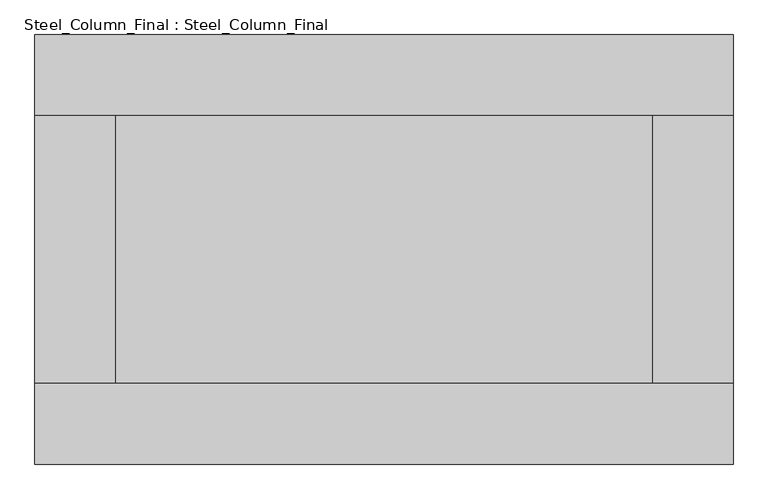
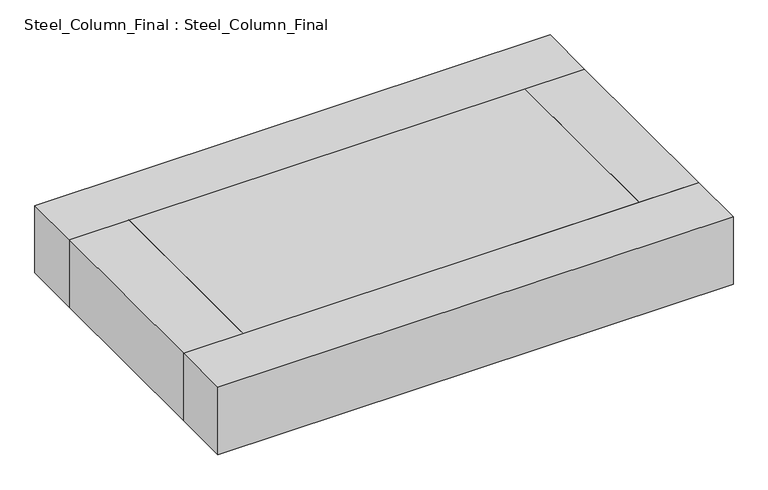
"""IFC4 building model written with IfcOpenShell, lengths in millimetres: proxy geometry, Steel_Column_Final : Steel_Column_Final."""

from ifc_helpers import new_model, si_unit, frame, origin, place, context, project, spatial, polyline, outline, extrude, source, transform, mapped, element, save


def steel_column_final_steel_column_final_ec0f6d93(model_context):
    return source(origin(), model_context, "Body", "SweptSolid", [
        extrude(outline(polyline([(6500.0, 2500.0), (-6500.0, 2500.0), (-6500.0, 4000.0), (6500.0, 4000.0), (6500.0, 2500.0)])), frame((0.0, 0.0, 83080.0), z_axis=(0.0, 0.0, 1.0), x_axis=(1.0, 0.0, 0.0)), (0.0, 0.0, 1.0), 1800.0),
        extrude(outline(polyline([(-6500.0, -2500.0), (6500.0, -2500.0), (6500.0, -4000.0), (-6500.0, -4000.0), (-6500.0, -2500.0)])), frame((0.0, 0.0, 83080.0), z_axis=(0.0, 0.0, 1.0), x_axis=(1.0, 0.0, 0.0)), (0.0, 0.0, 1.0), 1800.0),
        extrude(outline(polyline([(5000.0, -2500.0), (5000.0, 2500.0), (6500.0, 2500.0), (6500.0, -2500.0), (5000.0, -2500.0)])), frame((0.0, 0.0, 83080.0), z_axis=(0.0, 0.0, 1.0), x_axis=(1.0, 0.0, 0.0)), (0.0, 0.0, 1.0), 1800.0),
        extrude(outline(polyline([(-5000.0, 2500.0), (-5000.0, -2500.0), (-6500.0, -2500.0), (-6500.0, 2500.0), (-5000.0, 2500.0)])), frame((0.0, 0.0, 83080.0), z_axis=(0.0, 0.0, 1.0), x_axis=(1.0, 0.0, 0.0)), (0.0, 0.0, 1.0), 1800.0),
        extrude(outline(polyline([(-5000.0, -2500.0), (-5000.0, 2500.0), (5000.0, 2500.0), (5000.0, -2500.0), (-5000.0, -2500.0)])), frame((0.0, 0.0, 83080.0), z_axis=(0.0, 0.0, 1.0), x_axis=(1.0, 0.0, 0.0)), (0.0, 0.0, 1.0), 1800.0),
    ])


if __name__ == "__main__":
    model = new_model("IFC4")
    model_context = context("Model", 3, world=origin())
    ifc_project = project(units=[si_unit("LENGTHUNIT", "METRE", prefix="MILLI")], contexts=[model_context])
    site = spatial("IfcSite", under=ifc_project)
    building = spatial("IfcBuilding", under=site)
    placement = place(None, origin())
    steel_column_final_steel_column_final_shape = steel_column_final_steel_column_final_ec0f6d93(model_context)
    element("IfcBuildingElementProxy", 1, Name="Steel_Column_Final : Steel_Column_Final", ObjectType="Steel_Column_Final : Steel_Column_Final", at=placement, inside=building, context=model_context, shape_type="MappedRepresentation", body=[
        mapped(steel_column_final_steel_column_final_shape, transform((0.0, 0.0, 0.0), x_axis=(1.0, 0.0, 0.0), y_axis=(0.0, 1.0, 0.0), z_axis=(0.0, 0.0, 1.0))),
    ])
    save(model, "model.ifc")

# Revit data of these elements
# Type "Steel_Column_Final : Steel_Column_Final"
#   Top Width [instance default] = 5000 mm
#   Top Length = 10000 mm
#   Length = 21000 mm
#   Height [instance default] = 50000 mm
#   Bottom Width [instance default] = 5000 mm
#   Default Elevation = 0
# Element 1 (IfcBuildingElementProxy, "Steel_Column_Final : Steel_Column_Final")
#   Height = 83080 mm
